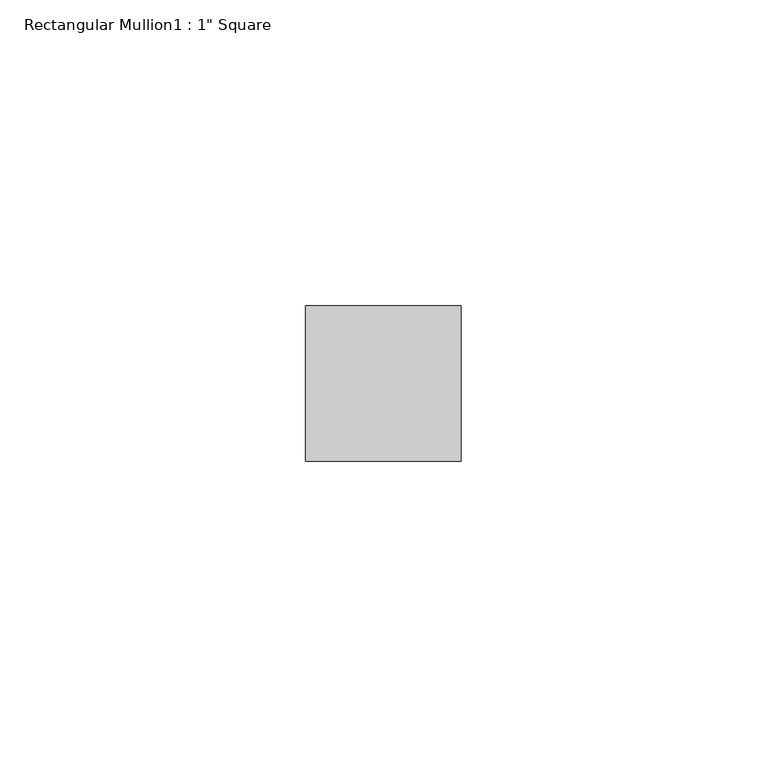
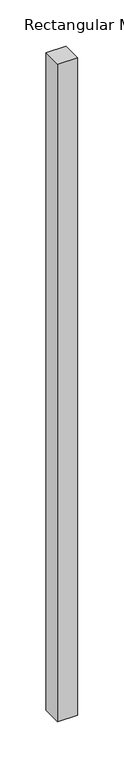
"""IFC4 building model written with IfcOpenShell, lengths in millimetres: member geometry."""

import ifcopenshell
import ifcopenshell.guid

model = None  # the IFC model being written
_history = None  # IfcOwnerHistory: only IFC2X3 demands one
_inside = {}  # id of a spatial element -> (the spatial element, [elements in it])
_under = {}  # id of a project, library or spatial element -> (it, [spatial elements below it])
_declared = {}  # id of a project -> (the project, [libraries it declares])
_typed = {}  # id of a type object -> (the type object, [elements of that type])
_made_of = {}  # id of a material, layer set ... -> (it, [elements and type objects made of it])


def new_model(schema):
    """Start an empty IFC model of exactly this schema.

    Asked for "IFC4X3", IfcOpenShell would pick the latest addendum, in which some entities
    have other attributes; the version numbers below select the first issue.
    IFC2X3 requires an IfcOwnerHistory on every rooted entity: one is made here for all.
    """
    global model, _history
    if schema == "IFC4X3":
        model = ifcopenshell.file(schema_version=(4, 3, 0, 0))
    else:
        model = ifcopenshell.file(schema=schema)
    _inside.clear()
    _under.clear()
    _declared.clear()
    _typed.clear()
    _made_of.clear()
    _history = None
    if model.schema == "IFC2X3":
        org = make("IfcOrganization", Name="unknown")
        user = make(
            "IfcPersonAndOrganization",
            ThePerson=make("IfcPerson", FamilyName="unknown"),
            TheOrganization=org,
        )
        app = make(
            "IfcApplication",
            ApplicationDeveloper=org,
            Version="unknown",
            ApplicationFullName="unknown",
            ApplicationIdentifier="unknown",
        )
        _history = make(
            "IfcOwnerHistory",
            OwningUser=user,
            OwningApplication=app,
            ChangeAction="ADDED",
            CreationDate=0,
        )
    return model


def make(cls, **values):
    """One entity of the class cls with the attributes given. An attribute that is None is left unset."""
    return model.create_entity(
        cls, **{name: value for name, value in values.items() if value is not None}
    )


def rooted(cls, **values):
    """An entity with a GlobalId (a new one), such as an element, a storey or a relation."""
    return make(cls, GlobalId=ifcopenshell.guid.new(), OwnerHistory=_history, **values)


def si_unit(unit_type, name, prefix=None):
    """IfcSIUnit, for example si_unit("LENGTHUNIT", "METRE", prefix="MILLI")."""
    return make("IfcSIUnit", UnitType=unit_type, Prefix=prefix, Name=name)


def assignment(units):
    """IfcUnitAssignment: the units of a project."""
    return None if units is None else make("IfcUnitAssignment", Units=units)


def point(xyz):
    """IfcCartesianPoint."""
    return None if xyz is None else make("IfcCartesianPoint", Coordinates=xyz)


def direction(xyz):
    """IfcDirection."""
    return None if xyz is None else make("IfcDirection", DirectionRatios=xyz)


def frame(location, z_axis=None, x_axis=None):
    """IfcAxis2Placement3D, a coordinate frame: its origin and axes. An axis left out is left unset."""
    return make(
        "IfcAxis2Placement3D",
        Location=point(location),
        Axis=direction(z_axis),
        RefDirection=direction(x_axis),
    )


def origin():
    """The frame at (0, 0, 0) with its axes left unset."""
    return frame((0.0, 0.0, 0.0))


def place(relative_to, where):
    """IfcLocalPlacement: puts the frame where relative to a parent placement (None: the world)."""
    return make(
        "IfcLocalPlacement", PlacementRelTo=relative_to, RelativePlacement=where
    )


def context(
    kind, dimensions, precision=None, world=None, true_north=None, identifier=None
):
    """IfcGeometricRepresentationContext, for example the 3D "Model" context."""
    return make(
        "IfcGeometricRepresentationContext",
        ContextIdentifier=identifier,
        ContextType=kind,
        CoordinateSpaceDimension=dimensions,
        Precision=precision,
        WorldCoordinateSystem=world,
        TrueNorth=true_north,
    )


def project(units=None, contexts=None):
    """IfcProject with its units and contexts."""
    return rooted(
        "IfcProject",
        Name="project",
        RepresentationContexts=contexts,
        UnitsInContext=assignment(units),
    )


def spatial(cls, under=None, at=None, **own):
    """A site, building, storey or space (cls), placed at a placement, below another one or the project."""
    s = rooted(cls, ObjectPlacement=at, **own)
    if under is not None:
        _under.setdefault(under.id(), (under, []))[1].append(s)
    return s


def polyline(points):
    """IfcPolyline through the points."""
    return make("IfcPolyline", Points=[point(p) for p in points])


def outline(outer, holes=None, kind="AREA"):
    """IfcArbitraryClosedProfileDef: a profile drawn as a closed curve; with holes, ...WithVoids."""
    if holes is None:
        return make("IfcArbitraryClosedProfileDef", ProfileType=kind, OuterCurve=outer)
    return make(
        "IfcArbitraryProfileDefWithVoids",
        ProfileType=kind,
        OuterCurve=outer,
        InnerCurves=holes,
    )


def extrude(swept, where, along, depth):
    """IfcExtrudedAreaSolid: the profile swept, set in the frame where, extruded along a direction by depth."""
    return make(
        "IfcExtrudedAreaSolid",
        SweptArea=swept,
        Position=where,
        ExtrudedDirection=direction(along),
        Depth=depth,
    )


def shape(context_of_items, identifier, shape_type, items):
    """IfcShapeRepresentation: the items that make up one representation, for example the "Body"."""
    return make(
        "IfcShapeRepresentation",
        ContextOfItems=context_of_items,
        RepresentationIdentifier=identifier,
        RepresentationType=shape_type,
        Items=items,
    )


def source(mapping_origin, context_of_items, identifier, shape_type, items):
    """IfcRepresentationMap: a shape defined once, which mapped items show again and again."""
    return make(
        "IfcRepresentationMap",
        MappingOrigin=mapping_origin,
        MappedRepresentation=shape(context_of_items, identifier, shape_type, items),
    )


def transform(
    local_origin,
    x_axis=None,
    y_axis=None,
    z_axis=None,
    scale=None,
    scale2=None,
    scale3=None,
    uniform=True,
):
    """IfcCartesianTransformationOperator3D, or its non-uniform kind. x_axis, y_axis, z_axis: its Axis1, 2, 3."""
    if uniform:
        return make(
            "IfcCartesianTransformationOperator3D",
            Axis1=direction(x_axis),
            Axis2=direction(y_axis),
            LocalOrigin=point(local_origin),
            Scale=scale,
            Axis3=direction(z_axis),
        )
    return make(
        "IfcCartesianTransformationOperator3DnonUniform",
        Axis1=direction(x_axis),
        Axis2=direction(y_axis),
        LocalOrigin=point(local_origin),
        Scale=scale,
        Axis3=direction(z_axis),
        Scale2=scale2,
        Scale3=scale3,
    )


def mapped(mapping_source, mapping_target):
    """IfcMappedItem: shows the shape of a source again, moved by a transform."""
    return make(
        "IfcMappedItem", MappingSource=mapping_source, MappingTarget=mapping_target
    )


def made_of(thing, what):
    """Note that an element or type object is made of a material, layer set ...; save() writes the relation."""
    if what is not None:
        _made_of.setdefault(what.id(), (what, []))[1].append(thing)
    return thing


def element(
    cls,
    number,
    at=None,
    inside=None,
    cuts=None,
    type_object=None,
    material=None,
    context=None,
    identifier="Body",
    shape_type=None,
    held_by="IfcProductDefinitionShape",
    body=None,
    shapes=None,
    **own,
):
    """One element of the class cls, such as IfcWall. Its Tag is "e" and its number.

    at: its placement. inside: the storey or other place that contains it. cuts: it is an
    opening in that element (IfcRelVoidsElement). A single representation is given by context,
    identifier, shape_type and body (its items); several are given by shapes. held_by: the class
    of the entity that holds the representations. save() writes the other relations.
    """
    e = rooted(cls, Tag="e%d" % number, ObjectPlacement=at, **own)
    if body is not None:
        shapes = [shape(context, identifier, shape_type, body)]
    if shapes is not None:
        e.Representation = make(held_by, Representations=shapes)
    if inside is not None:
        _inside.setdefault(inside.id(), (inside, []))[1].append(e)
    if cuts is not None:
        rooted(
            "IfcRelVoidsElement", RelatingBuildingElement=cuts, RelatedOpeningElement=e
        )
    if type_object is not None:
        _typed.setdefault(type_object.id(), (type_object, []))[1].append(e)
    return made_of(e, material)


def aggregate(whole, parts):
    """IfcRelAggregates: a whole, such as a stair, and the parts it consists of."""
    return rooted("IfcRelAggregates", RelatingObject=whole, RelatedObjects=parts)


def save(model, path):
    """Write the relations noted so far, then the file.

    IfcRelAggregates (storeys below a building ...), IfcRelContainedInSpatialStructure (elements
    in a storey), IfcRelDefinesByType, IfcRelAssociatesMaterial and IfcRelDeclares: one each for
    every whole, place, type object, material and project.
    """
    for whole, parts in _under.values():
        aggregate(whole, parts)
    for where, things in _inside.values():
        rooted(
            "IfcRelContainedInSpatialStructure",
            RelatedElements=things,
            RelatingStructure=where,
        )
    for kind, things in _typed.values():
        rooted("IfcRelDefinesByType", RelatedObjects=things, RelatingType=kind)
    for what, things in _made_of.values():
        rooted("IfcRelAssociatesMaterial", RelatedObjects=things, RelatingMaterial=what)
    for by, libraries in _declared.values():
        rooted("IfcRelDeclares", RelatingContext=by, RelatedDefinitions=libraries)
    model.write(path)


def member_fbd506e6(model_context):
    return source(origin(), model_context, "Body", "SweptSolid", [
        extrude(outline(polyline([(12.7, -19.05), (12.7, -44.45), (-12.7, -44.45), (-12.7, -19.05), (12.7, -19.05)])), frame((0.0, 0.0, -871.9298259), z_axis=(0.0, 0.0, 1.0), x_axis=(1.0, 0.0, 0.0)), (0.0, 0.0, 1.0), 871.9298259),
    ])


if __name__ == "__main__":
    model = new_model("IFC4")
    model_context = context("Model", 3, world=origin())
    ifc_project = project(units=[si_unit("LENGTHUNIT", "METRE", prefix="MILLI")], contexts=[model_context])
    site = spatial("IfcSite", under=ifc_project)
    building = spatial("IfcBuilding", under=site)
    placement = place(None, origin())
    member_shape = member_fbd506e6(model_context)
    element("IfcMember", 1, ObjectType="Rectangular Mullion1 : 1\" Square", at=placement, inside=building, context=model_context, shape_type="MappedRepresentation", body=[
        mapped(member_shape, transform((0.0, 0.0, 0.0), x_axis=(1.0, 0.0, 0.0), y_axis=(0.0, 1.0, 0.0), z_axis=(0.0, 0.0, 1.0))),
    ])
    save(model, "model.ifc")

# Revit data of these elements
# Type "Rectangular Mullion1 : 1\" Square"
#   built-in parameter 1007351 = 0.104167 (stored number, unit not read)
#   built-in parameter 1007304 = 0.0833333 (stored number, unit not read)
#   built-in parameter 1007301 = 0.0416667 (stored number, unit not read)
#   built-in parameter 1007300 = 0.0416667 (stored number, unit not read)
